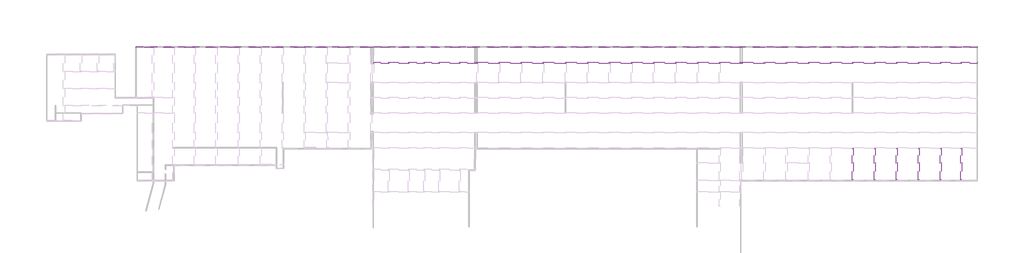
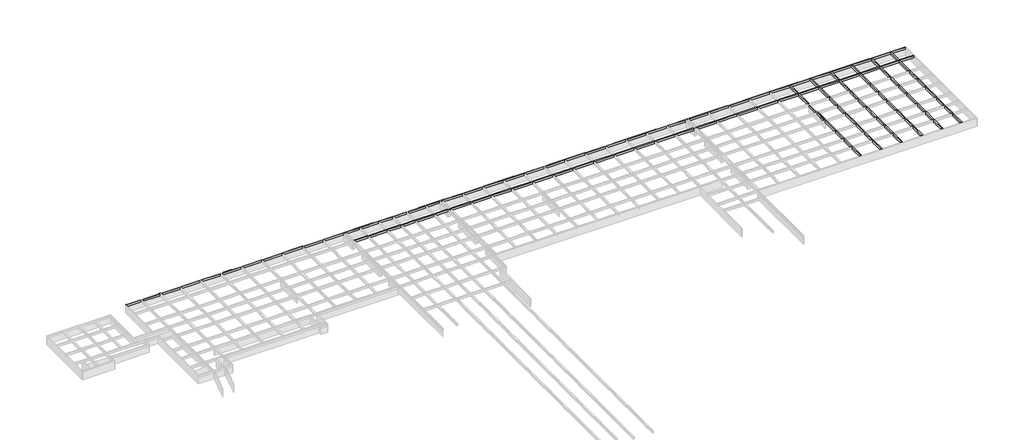
# One storey, part 14 of 14: 8 beams.
"""IFC4 building model written with IfcOpenShell, lengths in millimetres."""

import ifcopenshell
import ifcopenshell.guid

model = None  # the IFC model being written
_history = None  # IfcOwnerHistory: only IFC2X3 demands one
_inside = {}  # id of a spatial element -> (the spatial element, [elements in it])
_under = {}  # id of a project, library or spatial element -> (it, [spatial elements below it])
_declared = {}  # id of a project -> (the project, [libraries it declares])
_typed = {}  # id of a type object -> (the type object, [elements of that type])
_made_of = {}  # id of a material, layer set ... -> (it, [elements and type objects made of it])


def new_model(schema):
    """Start an empty IFC model of exactly this schema.

    Asked for "IFC4X3", IfcOpenShell would pick the latest addendum, in which some entities
    have other attributes; the version numbers below select the first issue.
    IFC2X3 requires an IfcOwnerHistory on every rooted entity: one is made here for all.
    """
    global model, _history
    if schema == "IFC4X3":
        model = ifcopenshell.file(schema_version=(4, 3, 0, 0))
    else:
        model = ifcopenshell.file(schema=schema)
    _inside.clear()
    _under.clear()
    _declared.clear()
    _typed.clear()
    _made_of.clear()
    _history = None
    if model.schema == "IFC2X3":
        org = make("IfcOrganization", Name="unknown")
        user = make(
            "IfcPersonAndOrganization",
            ThePerson=make("IfcPerson", FamilyName="unknown"),
            TheOrganization=org,
        )
        app = make(
            "IfcApplication",
            ApplicationDeveloper=org,
            Version="unknown",
            ApplicationFullName="unknown",
            ApplicationIdentifier="unknown",
        )
        _history = make(
            "IfcOwnerHistory",
            OwningUser=user,
            OwningApplication=app,
            ChangeAction="ADDED",
            CreationDate=0,
        )
    return model


def make(cls, **values):
    """One entity of the class cls with the attributes given. An attribute that is None is left unset."""
    return model.create_entity(
        cls, **{name: value for name, value in values.items() if value is not None}
    )


def rooted(cls, **values):
    """An entity with a GlobalId (a new one), such as an element, a storey or a relation."""
    return make(cls, GlobalId=ifcopenshell.guid.new(), OwnerHistory=_history, **values)


def si_unit(unit_type, name, prefix=None):
    """IfcSIUnit, for example si_unit("LENGTHUNIT", "METRE", prefix="MILLI")."""
    return make("IfcSIUnit", UnitType=unit_type, Prefix=prefix, Name=name)


def assignment(units):
    """IfcUnitAssignment: the units of a project."""
    return None if units is None else make("IfcUnitAssignment", Units=units)


def point(xyz):
    """IfcCartesianPoint."""
    return None if xyz is None else make("IfcCartesianPoint", Coordinates=xyz)


def direction(xyz):
    """IfcDirection."""
    return None if xyz is None else make("IfcDirection", DirectionRatios=xyz)


def frame(location, z_axis=None, x_axis=None):
    """IfcAxis2Placement3D, a coordinate frame: its origin and axes. An axis left out is left unset."""
    return make(
        "IfcAxis2Placement3D",
        Location=point(location),
        Axis=direction(z_axis),
        RefDirection=direction(x_axis),
    )


def origin():
    """The frame at (0, 0, 0) with its axes left unset."""
    return frame((0.0, 0.0, 0.0))


def place(relative_to, where):
    """IfcLocalPlacement: puts the frame where relative to a parent placement (None: the world)."""
    return make(
        "IfcLocalPlacement", PlacementRelTo=relative_to, RelativePlacement=where
    )


def context(
    kind, dimensions, precision=None, world=None, true_north=None, identifier=None
):
    """IfcGeometricRepresentationContext, for example the 3D "Model" context."""
    return make(
        "IfcGeometricRepresentationContext",
        ContextIdentifier=identifier,
        ContextType=kind,
        CoordinateSpaceDimension=dimensions,
        Precision=precision,
        WorldCoordinateSystem=world,
        TrueNorth=true_north,
    )


def project(units=None, contexts=None):
    """IfcProject with its units and contexts."""
    return rooted(
        "IfcProject",
        Name="project",
        RepresentationContexts=contexts,
        UnitsInContext=assignment(units),
    )


def spatial(cls, under=None, at=None, **own):
    """A site, building, storey or space (cls), placed at a placement, below another one or the project."""
    s = rooted(cls, ObjectPlacement=at, **own)
    if under is not None:
        _under.setdefault(under.id(), (under, []))[1].append(s)
    return s


def faces_of(points, faces, orient=None, outer=None):
    """IfcFace entities. A face is a list of loops; a loop is a list of indices into points, from 0.

    orient and outer hold one flag for each loop. By default every Orientation is true, the
    first loop of a face is its IfcFaceOuterBound and the others are IfcFaceBound.
    """
    made = []
    for i, loops in enumerate(faces):
        bounds = []
        for j, loop in enumerate(loops):
            is_outer = j == 0 if outer is None else outer[i][j]
            bounds.append(
                make(
                    "IfcFaceOuterBound" if is_outer else "IfcFaceBound",
                    Bound=make("IfcPolyLoop", Polygon=[points[k] for k in loop]),
                    Orientation=True if orient is None else orient[i][j],
                )
            )
        made.append(make("IfcFace", Bounds=bounds))
    return made


def faceted_brep(points, faces, orient=None, outer=None, voids=None):
    """IfcFacetedBrep: a solid bounded by flat faces; with voids (closed shells), ...WithVoids."""
    shared = [point(p) for p in points]
    hull = make("IfcClosedShell", CfsFaces=faces_of(shared, faces, orient, outer))
    if voids is None:
        return make("IfcFacetedBrep", Outer=hull)
    return make(
        "IfcFacetedBrepWithVoids",
        Outer=hull,
        Voids=[
            make(cls, CfsFaces=faces_of(shared, fs, o, b)) for cls, fs, o, b in voids
        ],
    )


def shape(context_of_items, identifier, shape_type, items):
    """IfcShapeRepresentation: the items that make up one representation, for example the "Body"."""
    return make(
        "IfcShapeRepresentation",
        ContextOfItems=context_of_items,
        RepresentationIdentifier=identifier,
        RepresentationType=shape_type,
        Items=items,
    )


def made_of(thing, what):
    """Note that an element or type object is made of a material, layer set ...; save() writes the relation."""
    if what is not None:
        _made_of.setdefault(what.id(), (what, []))[1].append(thing)
    return thing


def element(
    cls,
    number,
    at=None,
    inside=None,
    cuts=None,
    type_object=None,
    material=None,
    context=None,
    identifier="Body",
    shape_type=None,
    held_by="IfcProductDefinitionShape",
    body=None,
    shapes=None,
    **own,
):
    """One element of the class cls, such as IfcWall. Its Tag is "e" and its number.

    at: its placement. inside: the storey or other place that contains it. cuts: it is an
    opening in that element (IfcRelVoidsElement). A single representation is given by context,
    identifier, shape_type and body (its items); several are given by shapes. held_by: the class
    of the entity that holds the representations. save() writes the other relations.
    """
    e = rooted(cls, Tag="e%d" % number, ObjectPlacement=at, **own)
    if body is not None:
        shapes = [shape(context, identifier, shape_type, body)]
    if shapes is not None:
        e.Representation = make(held_by, Representations=shapes)
    if inside is not None:
        _inside.setdefault(inside.id(), (inside, []))[1].append(e)
    if cuts is not None:
        rooted(
            "IfcRelVoidsElement", RelatingBuildingElement=cuts, RelatedOpeningElement=e
        )
    if type_object is not None:
        _typed.setdefault(type_object.id(), (type_object, []))[1].append(e)
    return made_of(e, material)


def aggregate(whole, parts):
    """IfcRelAggregates: a whole, such as a stair, and the parts it consists of."""
    return rooted("IfcRelAggregates", RelatingObject=whole, RelatedObjects=parts)


def save(model, path):
    """Write the relations noted so far, then the file.

    IfcRelAggregates (storeys below a building ...), IfcRelContainedInSpatialStructure (elements
    in a storey), IfcRelDefinesByType, IfcRelAssociatesMaterial and IfcRelDeclares: one each for
    every whole, place, type object, material and project.
    """
    for whole, parts in _under.values():
        aggregate(whole, parts)
    for where, things in _inside.values():
        rooted(
            "IfcRelContainedInSpatialStructure",
            RelatedElements=things,
            RelatingStructure=where,
        )
    for kind, things in _typed.values():
        rooted("IfcRelDefinesByType", RelatedObjects=things, RelatingType=kind)
    for what, things in _made_of.values():
        rooted("IfcRelAssociatesMaterial", RelatedObjects=things, RelatingMaterial=what)
    for by, libraries in _declared.values():
        rooted("IfcRelDeclares", RelatingContext=by, RelatedDefinitions=libraries)
    model.write(path)


model = new_model("IFC4")

# Units and contexts
model_context = context("Model", 3, world=origin())
ifc_project = project(units=[si_unit("LENGTHUNIT", "METRE", prefix="MILLI")], contexts=[model_context])

# Site, building, storey
site = spatial("IfcSite", under=ifc_project)
building = spatial("IfcBuilding", under=site)
storey = spatial("IfcBuildingStorey", under=building, Name="户型图", Elevation=0.0)

# Beams
placement = place(None, origin())
element("IfcBeam", 1, ObjectType="混凝土 - 矩形梁 : KL_beam", at=placement, inside=storey, context=model_context, shape_type="Brep", body=[
    faceted_brep([(227227.2949044, -122797.8127788, 3300.0), (227227.2949044, -123197.8127788, 3300.0), (227227.2949044, -123197.8127788, 2500.0), (227227.2949044, -122797.8127788, 2500.0), (221727.2949044, -122797.8127788, 3300.0), (221327.2949044, -122797.8127788, 3300.0), (214491.1566028, -122797.8127788, 3300.0), (214091.1566028, -122797.8127788, 3300.0), (206763.3308695, -122797.8127788, 3300.0), (206363.3308695, -122797.8127788, 3300.0), (198949.6658892, -122797.8127788, 3300.0), (198549.6658892, -122797.8127788, 3300.0), (191137.2949044, -122797.8127788, 3300.0), (190737.2949044, -122797.8127788, 3300.0), (183327.7006088, -122797.8127788, 3300.0), (182927.7006088, -122797.8127788, 3300.0), (175558.5232577, -122797.8127788, 3300.0), (175158.5232577, -122797.8127788, 3300.0), (167740.9658811, -122797.8127788, 3300.0), (167340.9658811, -122797.8127788, 3300.0), (159907.8874304, -122797.8127788, 3300.0), (159507.8874304, -122797.8127788, 3300.0), (152140.9658811, -122797.8127788, 3300.0), (151740.9658811, -122797.8127788, 3300.0), (144337.2949044, -122797.8127788, 3300.0), (143937.2949044, -122797.8127788, 3300.0), (143577.2949044, -122797.8127788, 3300.0), (143177.2949044, -122797.8127788, 3300.0), (136347.2949044, -122797.8127788, 3300.0), (135947.2949044, -122797.8127788, 3300.0), (128527.2949044, -122797.8127788, 3300.0), (128127.2949044, -122797.8127788, 3300.0), (120717.7893795, -122797.8127788, 3300.0), (120317.7893795, -122797.8127788, 3300.0), (112927.2949044, -122797.8127788, 3300.0), (112527.2949044, -122797.8127788, 3300.0), (105157.0968236, -122797.8127788, 3300.0), (104757.0968236, -122797.8127788, 3300.0), (97322.1026691, -122797.8127788, 3300.0), (96922.1026691, -122797.8127788, 3300.0), (89602.2949044, -122797.8127788, 3300.0), (89202.2949044, -122797.8127788, 3300.0), (81802.2949044, -122797.8127788, 3300.0), (81402.2949044, -122797.8127788, 3300.0), (73867.4871398, -122797.8127788, 3300.0), (73467.4871398, -122797.8127788, 3300.0), (66130.1134745, -122797.8127788, 3300.0), (65730.1134745, -122797.8127788, 3300.0), (58330.1134745, -122797.8127788, 3300.0), (57930.1134745, -122797.8127788, 3300.0), (50537.2949044, -122797.8127788, 3300.0), (50137.2949044, -122797.8127788, 3300.0), (49716.5330009, -122797.8127788, 3300.0), (49316.5330009, -122797.8127788, 3300.0), (44331.9066405, -122797.8127788, 3300.0), (43931.9066405, -122797.8127788, 3300.0), (37081.5607309, -122797.8127788, 3300.0), (36681.5607309, -122797.8127788, 3300.0), (31751.9066405, -122797.8127788, 3300.0), (31351.9066405, -122797.8127788, 3300.0), (26321.5607309, -122797.8127788, 3300.0), (25921.5607309, -122797.8127788, 3300.0), (19160.0865653, -122797.8127788, 3300.0), (18760.0865653, -122797.8127788, 3300.0), (13677.2949044, -122797.8127788, 3300.0), (13677.2949044, -123197.8127788, 3300.0), (18760.0865653, -123197.8127788, 3300.0), (19160.0865653, -123197.8127788, 3300.0), (25921.5607309, -123197.8127788, 3300.0), (26321.5607309, -123197.8127788, 3300.0), (31351.9066405, -123197.8127788, 3300.0), (31751.9066405, -123197.8127788, 3300.0), (36681.5607309, -123197.8127788, 3300.0), (37081.5607309, -123197.8127788, 3300.0), (43931.9066405, -123197.8127788, 3300.0), (44331.9066405, -123197.8127788, 3300.0), (49316.5330009, -123197.8127788, 3300.0), (49716.5330009, -123197.8127788, 3300.0), (50137.2949044, -123197.8127788, 3300.0), (50537.2949044, -123197.8127788, 3300.0), (57930.1134745, -123197.8127788, 3300.0), (58330.1134745, -123197.8127788, 3300.0), (65730.1134745, -123197.8127788, 3300.0), (66130.1134745, -123197.8127788, 3300.0), (73467.4871398, -123197.8127788, 3300.0), (73867.4871398, -123197.8127788, 3300.0), (81402.2949044, -123197.8127788, 3300.0), (81802.2949044, -123197.8127788, 3300.0), (89202.2949044, -123197.8127788, 3300.0), (89602.2949044, -123197.8127788, 3300.0), (96922.1026691, -123197.8127788, 3300.0), (97322.1026691, -123197.8127788, 3300.0), (104757.0968236, -123197.8127788, 3300.0), (105157.0968236, -123197.8127788, 3300.0), (112527.2949044, -123197.8127788, 3300.0), (112927.2949044, -123197.8127788, 3300.0), (120317.7893795, -123197.8127788, 3300.0), (120717.7893795, -123197.8127788, 3300.0), (128127.2949044, -123197.8127788, 3300.0), (128527.2949044, -123197.8127788, 3300.0), (135947.2949044, -123197.8127788, 3300.0), (136347.2949044, -123197.8127788, 3300.0), (143177.2949044, -123197.8127788, 3300.0), (143577.2949044, -123197.8127788, 3300.0), (143937.2949044, -123197.8127788, 3300.0), (144337.2949044, -123197.8127788, 3300.0), (151740.9658811, -123197.8127788, 3300.0), (152140.9658811, -123197.8127788, 3300.0), (159507.8874304, -123197.8127788, 3300.0), (159907.8874304, -123197.8127788, 3300.0), (167340.9658811, -123197.8127788, 3300.0), (167740.9658811, -123197.8127788, 3300.0), (175158.5232577, -123197.8127788, 3300.0), (175558.5232577, -123197.8127788, 3300.0), (182927.7006088, -123197.8127788, 3300.0), (183327.7006088, -123197.8127788, 3300.0), (190737.2949044, -123197.8127788, 3300.0), (191137.2949044, -123197.8127788, 3300.0), (198549.6658892, -123197.8127788, 3300.0), (198949.6658892, -123197.8127788, 3300.0), (206363.3308695, -123197.8127788, 3300.0), (206763.3308695, -123197.8127788, 3300.0), (214091.1566028, -123197.8127788, 3300.0), (214491.1566028, -123197.8127788, 3300.0), (221327.2949044, -123197.8127788, 3300.0), (221727.2949044, -123197.8127788, 3300.0), (13677.2949044, -123197.8127788, 2500.0), (18760.0865653, -123197.8127788, 2500.0), (19160.0865653, -123197.8127788, 2500.0), (25921.5607309, -123197.8127788, 2500.0), (26321.5607309, -123197.8127788, 2500.0), (31351.9066405, -123197.8127788, 2500.0), (31751.9066405, -123197.8127788, 2500.0), (36681.5607309, -123197.8127788, 2500.0), (37081.5607309, -123197.8127788, 2500.0), (43931.9066405, -123197.8127788, 2500.0), (44331.9066405, -123197.8127788, 2500.0), (49316.5330009, -123197.8127788, 2500.0), (49716.5330009, -123197.8127788, 2500.0), (50137.2949044, -123197.8127788, 2500.0), (50537.2949044, -123197.8127788, 2500.0), (57930.1134745, -123197.8127788, 2500.0), (58330.1134745, -123197.8127788, 2500.0), (65730.1134745, -123197.8127788, 2500.0), (66130.1134745, -123197.8127788, 2500.0), (73467.4871398, -123197.8127788, 2500.0), (73867.4871398, -123197.8127788, 2500.0), (81402.2949044, -123197.8127788, 2500.0), (81802.2949044, -123197.8127788, 2500.0), (89202.2949044, -123197.8127788, 2500.0), (89602.2949044, -123197.8127788, 2500.0), (96922.1026691, -123197.8127788, 2500.0), (97322.1026691, -123197.8127788, 2500.0), (104757.0968236, -123197.8127788, 2500.0), (105157.0968236, -123197.8127788, 2500.0), (112527.2949044, -123197.8127788, 2500.0), (112927.2949044, -123197.8127788, 2500.0), (120317.7893795, -123197.8127788, 2500.0), (120717.7893795, -123197.8127788, 2500.0), (128127.2949044, -123197.8127788, 2500.0), (128527.2949044, -123197.8127788, 2500.0), (135947.2949044, -123197.8127788, 2500.0), (136347.2949044, -123197.8127788, 2500.0), (143177.2949044, -123197.8127788, 2500.0), (143577.2949044, -123197.8127788, 2500.0), (143937.2949044, -123197.8127788, 2500.0), (144337.2949044, -123197.8127788, 2500.0), (151740.9658811, -123197.8127788, 2500.0), (152140.9658811, -123197.8127788, 2500.0), (159507.8874304, -123197.8127788, 2500.0), (159907.8874304, -123197.8127788, 2500.0), (167340.9658811, -123197.8127788, 2500.0), (167740.9658811, -123197.8127788, 2500.0), (175158.5232577, -123197.8127788, 2500.0), (175558.5232577, -123197.8127788, 2500.0), (182927.7006088, -123197.8127788, 2500.0), (183327.7006088, -123197.8127788, 2500.0), (190737.2949044, -123197.8127788, 2500.0), (191137.2949044, -123197.8127788, 2500.0), (198549.6658892, -123197.8127788, 2500.0), (198949.6658892, -123197.8127788, 2500.0), (206363.3308695, -123197.8127788, 2500.0), (206763.3308695, -123197.8127788, 2500.0), (214091.1566028, -123197.8127788, 2500.0), (214491.1566028, -123197.8127788, 2500.0), (221327.2949044, -123197.8127788, 2500.0), (221727.2949044, -123197.8127788, 2500.0), (13677.2949044, -122797.8127788, 2500.0), (18760.0865653, -122797.8127788, 2500.0), (19160.0865653, -122797.8127788, 2500.0), (25921.5607309, -122797.8127788, 2500.0), (26321.5607309, -122797.8127788, 2500.0), (31351.9066405, -122797.8127788, 2500.0), (31751.9066405, -122797.8127788, 2500.0), (36681.5607309, -122797.8127788, 2500.0), (37081.5607309, -122797.8127788, 2500.0), (43931.9066405, -122797.8127788, 2500.0), (44331.9066405, -122797.8127788, 2500.0), (49316.5330009, -122797.8127788, 2500.0), (49716.5330009, -122797.8127788, 2500.0), (50137.2949044, -122797.8127788, 2500.0), (50537.2949044, -122797.8127788, 2500.0), (57930.1134745, -122797.8127788, 2500.0), (58330.1134745, -122797.8127788, 2500.0), (65730.1134745, -122797.8127788, 2500.0), (66130.1134745, -122797.8127788, 2500.0), (73467.4871398, -122797.8127788, 2500.0), (73867.4871398, -122797.8127788, 2500.0), (81402.2949044, -122797.8127788, 2500.0), (81802.2949044, -122797.8127788, 2500.0), (89202.2949044, -122797.8127788, 2500.0), (89602.2949044, -122797.8127788, 2500.0), (96922.1026691, -122797.8127788, 2500.0), (97322.1026691, -122797.8127788, 2500.0), (104757.0968236, -122797.8127788, 2500.0), (105157.0968236, -122797.8127788, 2500.0), (112527.2949044, -122797.8127788, 2500.0), (112927.2949044, -122797.8127788, 2500.0), (120317.7893795, -122797.8127788, 2500.0), (120717.7893795, -122797.8127788, 2500.0), (128127.2949044, -122797.8127788, 2500.0), (128527.2949044, -122797.8127788, 2500.0), (135947.2949044, -122797.8127788, 2500.0), (136347.2949044, -122797.8127788, 2500.0), (143177.2949044, -122797.8127788, 2500.0), (143577.2949044, -122797.8127788, 2500.0), (143937.2949044, -122797.8127788, 2500.0), (144337.2949044, -122797.8127788, 2500.0), (151740.9658811, -122797.8127788, 2500.0), (152140.9658811, -122797.8127788, 2500.0), (159507.8874304, -122797.8127788, 2500.0), (159907.8874304, -122797.8127788, 2500.0), (167340.9658811, -122797.8127788, 2500.0), (167740.9658811, -122797.8127788, 2500.0), (175158.5232577, -122797.8127788, 2500.0), (175558.5232577, -122797.8127788, 2500.0), (182927.7006088, -122797.8127788, 2500.0), (183327.7006088, -122797.8127788, 2500.0), (190737.2949044, -122797.8127788, 2500.0), (191137.2949044, -122797.8127788, 2500.0), (198549.6658892, -122797.8127788, 2500.0), (198949.6658892, -122797.8127788, 2500.0), (206363.3308695, -122797.8127788, 2500.0), (206763.3308695, -122797.8127788, 2500.0), (214091.1566028, -122797.8127788, 2500.0), (214491.1566028, -122797.8127788, 2500.0), (221327.2949044, -122797.8127788, 2500.0), (221727.2949044, -122797.8127788, 2500.0)], [[[0, 1, 2, 3]], [[1, 0, 4, 5, 6, 7, 8, 9, 10, 11, 12, 13, 14, 15, 16, 17, 18, 19, 20, 21, 22, 23, 24, 25, 26, 27, 28, 29, 30, 31, 32, 33, 34, 35, 36, 37, 38, 39, 40, 41, 42, 43, 44, 45, 46, 47, 48, 49, 50, 51, 52, 53, 54, 55, 56, 57, 58, 59, 60, 61, 62, 63, 64, 65, 66, 67, 68, 69, 70, 71, 72, 73, 74, 75, 76, 77, 78, 79, 80, 81, 82, 83, 84, 85, 86, 87, 88, 89, 90, 91, 92, 93, 94, 95, 96, 97, 98, 99, 100, 101, 102, 103, 104, 105, 106, 107, 108, 109, 110, 111, 112, 113, 114, 115, 116, 117, 118, 119, 120, 121, 122, 123, 124, 125]], [[2, 1, 125, 124, 123, 122, 121, 120, 119, 118, 117, 116, 115, 114, 113, 112, 111, 110, 109, 108, 107, 106, 105, 104, 103, 102, 101, 100, 99, 98, 97, 96, 95, 94, 93, 92, 91, 90, 89, 88, 87, 86, 85, 84, 83, 82, 81, 80, 79, 78, 77, 76, 75, 74, 73, 72, 71, 70, 69, 68, 67, 66, 65, 126, 127, 128, 129, 130, 131, 132, 133, 134, 135, 136, 137, 138, 139, 140, 141, 142, 143, 144, 145, 146, 147, 148, 149, 150, 151, 152, 153, 154, 155, 156, 157, 158, 159, 160, 161, 162, 163, 164, 165, 166, 167, 168, 169, 170, 171, 172, 173, 174, 175, 176, 177, 178, 179, 180, 181, 182, 183, 184, 185, 186]], [[3, 2, 186, 185, 184, 183, 182, 181, 180, 179, 178, 177, 176, 175, 174, 173, 172, 171, 170, 169, 168, 167, 166, 165, 164, 163, 162, 161, 160, 159, 158, 157, 156, 155, 154, 153, 152, 151, 150, 149, 148, 147, 146, 145, 144, 143, 142, 141, 140, 139, 138, 137, 136, 135, 134, 133, 132, 131, 130, 129, 128, 127, 126, 187, 188, 189, 190, 191, 192, 193, 194, 195, 196, 197, 198, 199, 200, 201, 202, 203, 204, 205, 206, 207, 208, 209, 210, 211, 212, 213, 214, 215, 216, 217, 218, 219, 220, 221, 222, 223, 224, 225, 226, 227, 228, 229, 230, 231, 232, 233, 234, 235, 236, 237, 238, 239, 240, 241, 242, 243, 244, 245, 246, 247]], [[0, 3, 247, 246, 245, 244, 243, 242, 241, 240, 239, 238, 237, 236, 235, 234, 233, 232, 231, 230, 229, 228, 227, 226, 225, 224, 223, 222, 221, 220, 219, 218, 217, 216, 215, 214, 213, 212, 211, 210, 209, 208, 207, 206, 205, 204, 203, 202, 201, 200, 199, 198, 197, 196, 195, 194, 193, 192, 191, 190, 189, 188, 187, 64, 63, 62, 61, 60, 59, 58, 57, 56, 55, 54, 53, 52, 51, 50, 49, 48, 47, 46, 45, 44, 43, 42, 41, 40, 39, 38, 37, 36, 35, 34, 33, 32, 31, 30, 29, 28, 27, 26, 25, 24, 23, 22, 21, 20, 19, 18, 17, 16, 15, 14, 13, 12, 11, 10, 9, 8, 7, 6, 5, 4]], [[65, 64, 187, 126]]]),
])
element("IfcBeam", 2, ObjectType="混凝土 - 矩形梁 : KL_beam", at=placement, inside=storey, context=model_context, shape_type="Brep", body=[
    faceted_brep([(182927.7006088, -122797.8127788, 3300.0), (183327.7006088, -122797.8127788, 3300.0), (183327.7006088, -117558.950757, 3300.0), (182927.7006088, -117558.950757, 3300.0), (182927.7006088, -122797.8127788, 2500.0), (182927.7006088, -117558.950757, 2500.0), (183327.7006088, -122797.8127788, 2500.0), (183327.7006088, -117558.950757, 2500.0)], [[[0, 1, 2, 3]], [[4, 0, 3, 5]], [[6, 4, 5, 7]], [[1, 6, 7, 2]], [[1, 0, 4, 6]], [[3, 2, 7, 5]]]),
    faceted_brep([(182927.7006088, -123197.8127788, 3300.0), (183327.7006088, -123197.8127788, 3300.0), (183327.7006088, -123197.8127788, 2500.0), (182927.7006088, -123197.8127788, 2500.0), (183327.7006088, -129780.0179086, 3300.0), (182927.7006088, -129780.0179086, 3300.0), (182927.7006088, -129780.0179086, 2500.0), (183327.7006088, -129780.0179086, 2500.0)], [[[0, 1, 2, 3]], [[4, 5, 6, 7]], [[1, 0, 5, 4]], [[0, 3, 6, 5]], [[3, 2, 7, 6]], [[2, 1, 4, 7]]]),
    faceted_brep([(183327.7006088, -130180.0179086, 3300.0), (182927.7006088, -130180.0179086, 3300.0), (182927.7006088, -135180.0179086, 3300.0), (183327.7006088, -135180.0179086, 3300.0), (182927.7006088, -130180.0179086, 2500.0), (182927.7006088, -135180.0179086, 2500.0), (183327.7006088, -130180.0179086, 2500.0), (183327.7006088, -135180.0179086, 2500.0)], [[[0, 1, 2, 3]], [[1, 4, 5, 2]], [[4, 6, 7, 5]], [[6, 0, 3, 7]], [[1, 0, 6, 4]], [[3, 2, 5, 7]]]),
    faceted_brep([(182927.7006088, -135580.0179086, 3300.0), (183327.7006088, -135580.0179086, 3300.0), (183327.7006088, -135580.0179086, 2500.0), (182927.7006088, -135580.0179086, 2500.0), (183327.7006088, -140520.0179086, 3300.0), (182927.7006088, -140520.0179086, 3300.0), (182927.7006088, -140520.0179086, 2500.0), (183327.7006088, -140520.0179086, 2500.0)], [[[0, 1, 2, 3]], [[4, 5, 6, 7]], [[1, 0, 5, 4]], [[0, 3, 6, 5]], [[3, 2, 7, 6]], [[2, 1, 4, 7]]]),
    faceted_brep([(182927.7006088, -140920.0179086, 3300.0), (183327.7006088, -140920.0179086, 3300.0), (183327.7006088, -140920.0179086, 2500.0), (182927.7006088, -140920.0179086, 2500.0), (183327.7006088, -147499.284307, 3300.0), (182927.7006088, -147499.284307, 3300.0), (182927.7006088, -147499.284307, 2500.0), (183327.7006088, -147499.284307, 2500.0)], [[[0, 1, 2, 3]], [[4, 5, 6, 7]], [[1, 0, 5, 4]], [[0, 3, 6, 5]], [[3, 2, 7, 6]], [[2, 1, 4, 7]]]),
    faceted_brep([(182927.7006088, -147899.284307, 3300.0), (183327.7006088, -147899.284307, 3300.0), (183327.7006088, -147899.284307, 2500.0), (182927.7006088, -147899.284307, 2500.0), (183327.7006088, -152899.284307, 3300.0), (182927.7006088, -152899.284307, 3300.0), (182927.7006088, -152899.284307, 2500.0), (183327.7006088, -152899.284307, 2500.0)], [[[0, 1, 2, 3]], [[4, 5, 6, 7]], [[1, 0, 5, 4]], [[0, 3, 6, 5]], [[3, 2, 7, 6]], [[2, 1, 4, 7]]]),
    faceted_brep([(182927.7006088, -153299.284307, 3300.0), (183327.7006088, -153299.284307, 3300.0), (183327.7006088, -153299.284307, 2500.0), (182927.7006088, -153299.284307, 2500.0), (183327.7006088, -164396.0449275, 3300.0), (182927.7006088, -164396.0449275, 3300.0), (182927.7006088, -164396.0449275, 2500.0), (183327.7006088, -164396.0449275, 2500.0), (182927.7006088, -158198.950757, 3300.0), (182927.7006088, -158598.950757, 3300.0), (183327.7006088, -158598.950757, 3300.0), (183327.7006088, -158198.950757, 3300.0), (182927.7006088, -158198.950757, 2500.0), (182927.7006088, -158598.950757, 2500.0), (183327.7006088, -158198.950757, 2500.0), (183327.7006088, -158598.950757, 2500.0)], [[[0, 1, 2, 3]], [[4, 5, 6, 7]], [[1, 0, 8, 9, 5, 4, 10, 11]], [[0, 3, 12, 13, 6, 5, 9, 8]], [[3, 2, 14, 15, 7, 6, 13, 12]], [[2, 1, 11, 10, 4, 7, 15, 14]]]),
])
element("IfcBeam", 3, ObjectType="混凝土 - 矩形梁 : KL_beam", at=placement, inside=storey, context=model_context, shape_type="Brep", body=[
    faceted_brep([(191137.2949044, -153299.284307, 3300.0), (190737.2949044, -153299.284307, 3300.0), (190737.2949044, -158198.950757, 3300.0), (190737.2949044, -158598.950757, 3300.0), (190737.2949044, -164396.0449275, 3300.0), (191137.2949044, -164396.0449275, 3300.0), (191137.2949044, -158598.950757, 3300.0), (191137.2949044, -158198.950757, 3300.0), (191137.2949044, -153299.284307, 2500.0), (191137.2949044, -164396.0449275, 2500.0), (191137.2949044, -158598.950757, 2500.0), (191137.2949044, -158198.950757, 2500.0), (190737.2949044, -153299.284307, 2500.0), (190737.2949044, -164396.0449275, 2500.0), (190737.2949044, -158598.950757, 2500.0), (190737.2949044, -158198.950757, 2500.0)], [[[0, 1, 2, 3, 4, 5, 6, 7]], [[8, 0, 7, 6, 5, 9, 10, 11]], [[12, 8, 11, 10, 9, 13, 14, 15]], [[1, 12, 15, 14, 13, 4, 3, 2]], [[1, 0, 8, 12]], [[5, 4, 13, 9]]]),
    faceted_brep([(190737.2949044, -123197.8127788, 3300.0), (191137.2949044, -123197.8127788, 3300.0), (191137.2949044, -123197.8127788, 2500.0), (190737.2949044, -123197.8127788, 2500.0), (191137.2949044, -129780.0179086, 3300.0), (190737.2949044, -129780.0179086, 3300.0), (190737.2949044, -129780.0179086, 2500.0), (191137.2949044, -129780.0179086, 2500.0)], [[[0, 1, 2, 3]], [[4, 5, 6, 7]], [[1, 0, 5, 4]], [[2, 1, 4, 7]], [[3, 2, 7, 6]], [[0, 3, 6, 5]]]),
    faceted_brep([(191137.2949044, -122797.8127788, 3300.0), (190737.2949044, -122797.8127788, 3300.0), (190737.2949044, -122797.8127788, 2500.0), (191137.2949044, -122797.8127788, 2500.0), (191137.2949044, -117558.950757, 3300.0), (190737.2949044, -117558.950757, 3300.0), (191137.2949044, -117558.950757, 2500.0), (190737.2949044, -117558.950757, 2500.0)], [[[0, 1, 2, 3]], [[1, 0, 4, 5]], [[0, 3, 6, 4]], [[3, 2, 7, 6]], [[2, 1, 5, 7]], [[5, 4, 6, 7]]]),
    faceted_brep([(190737.2949044, -130180.0179086, 3300.0), (191137.2949044, -130180.0179086, 3300.0), (191137.2949044, -130180.0179086, 2500.0), (190737.2949044, -130180.0179086, 2500.0), (191137.2949044, -135180.0179086, 3300.0), (190737.2949044, -135180.0179086, 3300.0), (190737.2949044, -135180.0179086, 2500.0), (191137.2949044, -135180.0179086, 2500.0)], [[[0, 1, 2, 3]], [[4, 5, 6, 7]], [[1, 0, 5, 4]], [[2, 1, 4, 7]], [[3, 2, 7, 6]], [[0, 3, 6, 5]]]),
    faceted_brep([(190737.2949044, -135580.0179086, 3300.0), (191137.2949044, -135580.0179086, 3300.0), (191137.2949044, -135580.0179086, 2500.0), (190737.2949044, -135580.0179086, 2500.0), (191137.2949044, -140520.0179086, 3300.0), (190737.2949044, -140520.0179086, 3300.0), (190737.2949044, -140520.0179086, 2500.0), (191137.2949044, -140520.0179086, 2500.0)], [[[0, 1, 2, 3]], [[4, 5, 6, 7]], [[1, 0, 5, 4]], [[2, 1, 4, 7]], [[3, 2, 7, 6]], [[0, 3, 6, 5]]]),
    faceted_brep([(190737.2949044, -140920.0179086, 3300.0), (191137.2949044, -140920.0179086, 3300.0), (191137.2949044, -140920.0179086, 2500.0), (190737.2949044, -140920.0179086, 2500.0), (191137.2949044, -147499.284307, 3300.0), (190737.2949044, -147499.284307, 3300.0), (190737.2949044, -147499.284307, 2500.0), (191137.2949044, -147499.284307, 2500.0)], [[[0, 1, 2, 3]], [[4, 5, 6, 7]], [[1, 0, 5, 4]], [[2, 1, 4, 7]], [[3, 2, 7, 6]], [[0, 3, 6, 5]]]),
    faceted_brep([(190737.2949044, -147899.284307, 3300.0), (191137.2949044, -147899.284307, 3300.0), (191137.2949044, -147899.284307, 2500.0), (190737.2949044, -147899.284307, 2500.0), (191137.2949044, -152899.284307, 3300.0), (190737.2949044, -152899.284307, 3300.0), (190737.2949044, -152899.284307, 2500.0), (191137.2949044, -152899.284307, 2500.0)], [[[0, 1, 2, 3]], [[4, 5, 6, 7]], [[1, 0, 5, 4]], [[2, 1, 4, 7]], [[3, 2, 7, 6]], [[0, 3, 6, 5]]]),
])
element("IfcBeam", 4, ObjectType="混凝土 - 矩形梁 : KL_beam", at=placement, inside=storey, context=model_context, shape_type="Brep", body=[
    faceted_brep([(198549.6658892, -122797.8127788, 3300.0), (198949.6658892, -122797.8127788, 3300.0), (198949.6658892, -117558.950757, 3300.0), (198549.6658892, -117558.950757, 3300.0), (198549.6658892, -122797.8127788, 2500.0), (198549.6658892, -117558.950757, 2500.0), (198949.6658892, -122797.8127788, 2500.0), (198949.6658892, -117558.950757, 2500.0)], [[[0, 1, 2, 3]], [[4, 0, 3, 5]], [[6, 4, 5, 7]], [[1, 6, 7, 2]], [[1, 0, 4, 6]], [[3, 2, 7, 5]]]),
    faceted_brep([(198549.6658892, -123197.8127788, 3300.0), (198949.6658892, -123197.8127788, 3300.0), (198949.6658892, -123197.8127788, 2500.0), (198549.6658892, -123197.8127788, 2500.0), (198949.6658892, -129780.0179086, 3300.0), (198549.6658892, -129780.0179086, 3300.0), (198549.6658892, -129780.0179086, 2500.0), (198949.6658892, -129780.0179086, 2500.0)], [[[0, 1, 2, 3]], [[4, 5, 6, 7]], [[1, 0, 5, 4]], [[0, 3, 6, 5]], [[3, 2, 7, 6]], [[2, 1, 4, 7]]]),
    faceted_brep([(198949.6658892, -130180.0179086, 3300.0), (198549.6658892, -130180.0179086, 3300.0), (198549.6658892, -135180.0179086, 3300.0), (198949.6658892, -135180.0179086, 3300.0), (198549.6658892, -130180.0179086, 2500.0), (198549.6658892, -135180.0179086, 2500.0), (198949.6658892, -130180.0179086, 2500.0), (198949.6658892, -135180.0179086, 2500.0)], [[[0, 1, 2, 3]], [[1, 4, 5, 2]], [[4, 6, 7, 5]], [[6, 0, 3, 7]], [[1, 0, 6, 4]], [[3, 2, 5, 7]]]),
    faceted_brep([(198549.6658892, -135580.0179086, 3300.0), (198949.6658892, -135580.0179086, 3300.0), (198949.6658892, -135580.0179086, 2500.0), (198549.6658892, -135580.0179086, 2500.0), (198949.6658892, -140520.0179086, 3300.0), (198549.6658892, -140520.0179086, 3300.0), (198549.6658892, -140520.0179086, 2500.0), (198949.6658892, -140520.0179086, 2500.0)], [[[0, 1, 2, 3]], [[4, 5, 6, 7]], [[1, 0, 5, 4]], [[0, 3, 6, 5]], [[3, 2, 7, 6]], [[2, 1, 4, 7]]]),
    faceted_brep([(198549.6658892, -140920.0179086, 3300.0), (198949.6658892, -140920.0179086, 3300.0), (198949.6658892, -140920.0179086, 2500.0), (198549.6658892, -140920.0179086, 2500.0), (198949.6658892, -147499.284307, 3300.0), (198549.6658892, -147499.284307, 3300.0), (198549.6658892, -147499.284307, 2500.0), (198949.6658892, -147499.284307, 2500.0)], [[[0, 1, 2, 3]], [[4, 5, 6, 7]], [[1, 0, 5, 4]], [[0, 3, 6, 5]], [[3, 2, 7, 6]], [[2, 1, 4, 7]]]),
    faceted_brep([(198549.6658892, -147899.284307, 3300.0), (198949.6658892, -147899.284307, 3300.0), (198949.6658892, -147899.284307, 2500.0), (198549.6658892, -147899.284307, 2500.0), (198949.6658892, -152899.284307, 3300.0), (198549.6658892, -152899.284307, 3300.0), (198549.6658892, -152899.284307, 2500.0), (198949.6658892, -152899.284307, 2500.0)], [[[0, 1, 2, 3]], [[4, 5, 6, 7]], [[1, 0, 5, 4]], [[0, 3, 6, 5]], [[3, 2, 7, 6]], [[2, 1, 4, 7]]]),
    faceted_brep([(198549.6658892, -153299.284307, 3300.0), (198949.6658892, -153299.284307, 3300.0), (198949.6658892, -153299.284307, 2500.0), (198549.6658892, -153299.284307, 2500.0), (198949.6658892, -164396.0449275, 3300.0), (198549.6658892, -164396.0449275, 3300.0), (198549.6658892, -164396.0449275, 2500.0), (198949.6658892, -164396.0449275, 2500.0), (198549.6658892, -158198.950757, 3300.0), (198549.6658892, -158598.950757, 3300.0), (198949.6658892, -158598.950757, 3300.0), (198949.6658892, -158198.950757, 3300.0), (198549.6658892, -158198.950757, 2500.0), (198549.6658892, -158598.950757, 2500.0), (198949.6658892, -158198.950757, 2500.0), (198949.6658892, -158598.950757, 2500.0)], [[[0, 1, 2, 3]], [[4, 5, 6, 7]], [[1, 0, 8, 9, 5, 4, 10, 11]], [[0, 3, 12, 13, 6, 5, 9, 8]], [[3, 2, 14, 15, 7, 6, 13, 12]], [[2, 1, 11, 10, 4, 7, 15, 14]]]),
])
element("IfcBeam", 5, ObjectType="混凝土 - 矩形梁 : KL_beam", at=placement, inside=storey, context=model_context, shape_type="Brep", body=[
    faceted_brep([(206763.3308695, -153299.284307, 3300.0), (206363.3308695, -153299.284307, 3300.0), (206363.3308695, -158198.950757, 3300.0), (206363.3308695, -158598.950757, 3300.0), (206363.3308695, -164396.0449275, 3300.0), (206763.3308695, -164396.0449275, 3300.0), (206763.3308695, -158598.950757, 3300.0), (206763.3308695, -158198.950757, 3300.0), (206763.3308695, -153299.284307, 2500.0), (206763.3308695, -164396.0449275, 2500.0), (206763.3308695, -158598.950757, 2500.0), (206763.3308695, -158198.950757, 2500.0), (206363.3308695, -153299.284307, 2500.0), (206363.3308695, -164396.0449275, 2500.0), (206363.3308695, -158598.950757, 2500.0), (206363.3308695, -158198.950757, 2500.0)], [[[0, 1, 2, 3, 4, 5, 6, 7]], [[8, 0, 7, 6, 5, 9, 10, 11]], [[12, 8, 11, 10, 9, 13, 14, 15]], [[1, 12, 15, 14, 13, 4, 3, 2]], [[1, 0, 8, 12]], [[5, 4, 13, 9]]]),
    faceted_brep([(206363.3308695, -123197.8127788, 3300.0), (206763.3308695, -123197.8127788, 3300.0), (206763.3308695, -123197.8127788, 2500.0), (206363.3308695, -123197.8127788, 2500.0), (206763.3308695, -129780.0179086, 3300.0), (206363.3308695, -129780.0179086, 3300.0), (206363.3308695, -129780.0179086, 2500.0), (206763.3308695, -129780.0179086, 2500.0)], [[[0, 1, 2, 3]], [[4, 5, 6, 7]], [[1, 0, 5, 4]], [[2, 1, 4, 7]], [[3, 2, 7, 6]], [[0, 3, 6, 5]]]),
    faceted_brep([(206763.3308695, -122797.8127788, 3300.0), (206363.3308695, -122797.8127788, 3300.0), (206363.3308695, -122797.8127788, 2500.0), (206763.3308695, -122797.8127788, 2500.0), (206763.3308695, -117558.950757, 3300.0), (206363.3308695, -117558.950757, 3300.0), (206763.3308695, -117558.950757, 2500.0), (206363.3308695, -117558.950757, 2500.0)], [[[0, 1, 2, 3]], [[1, 0, 4, 5]], [[0, 3, 6, 4]], [[3, 2, 7, 6]], [[2, 1, 5, 7]], [[5, 4, 6, 7]]]),
    faceted_brep([(206363.3308695, -130180.0179086, 3300.0), (206763.3308695, -130180.0179086, 3300.0), (206763.3308695, -130180.0179086, 2500.0), (206363.3308695, -130180.0179086, 2500.0), (206763.3308695, -135180.0179086, 3300.0), (206363.3308695, -135180.0179086, 3300.0), (206363.3308695, -135180.0179086, 2500.0), (206763.3308695, -135180.0179086, 2500.0)], [[[0, 1, 2, 3]], [[4, 5, 6, 7]], [[1, 0, 5, 4]], [[2, 1, 4, 7]], [[3, 2, 7, 6]], [[0, 3, 6, 5]]]),
    faceted_brep([(206363.3308695, -135580.0179086, 3300.0), (206763.3308695, -135580.0179086, 3300.0), (206763.3308695, -135580.0179086, 2500.0), (206363.3308695, -135580.0179086, 2500.0), (206763.3308695, -140520.0179086, 3300.0), (206363.3308695, -140520.0179086, 3300.0), (206363.3308695, -140520.0179086, 2500.0), (206763.3308695, -140520.0179086, 2500.0)], [[[0, 1, 2, 3]], [[4, 5, 6, 7]], [[1, 0, 5, 4]], [[2, 1, 4, 7]], [[3, 2, 7, 6]], [[0, 3, 6, 5]]]),
    faceted_brep([(206363.3308695, -140920.0179086, 3300.0), (206763.3308695, -140920.0179086, 3300.0), (206763.3308695, -140920.0179086, 2500.0), (206363.3308695, -140920.0179086, 2500.0), (206763.3308695, -147499.284307, 3300.0), (206363.3308695, -147499.284307, 3300.0), (206363.3308695, -147499.284307, 2500.0), (206763.3308695, -147499.284307, 2500.0)], [[[0, 1, 2, 3]], [[4, 5, 6, 7]], [[1, 0, 5, 4]], [[2, 1, 4, 7]], [[3, 2, 7, 6]], [[0, 3, 6, 5]]]),
    faceted_brep([(206363.3308695, -147899.284307, 3300.0), (206763.3308695, -147899.284307, 3300.0), (206763.3308695, -147899.284307, 2500.0), (206363.3308695, -147899.284307, 2500.0), (206763.3308695, -152899.284307, 3300.0), (206363.3308695, -152899.284307, 3300.0), (206363.3308695, -152899.284307, 2500.0), (206763.3308695, -152899.284307, 2500.0)], [[[0, 1, 2, 3]], [[4, 5, 6, 7]], [[1, 0, 5, 4]], [[2, 1, 4, 7]], [[3, 2, 7, 6]], [[0, 3, 6, 5]]]),
])
element("IfcBeam", 6, ObjectType="混凝土 - 矩形梁 : KL_beam", at=placement, inside=storey, context=model_context, shape_type="Brep", body=[
    faceted_brep([(214091.1566028, -122797.8127788, 3300.0), (214491.1566028, -122797.8127788, 3300.0), (214491.1566028, -117558.950757, 3300.0), (214091.1566028, -117558.950757, 3300.0), (214091.1566028, -122797.8127788, 2500.0), (214091.1566028, -117558.950757, 2500.0), (214491.1566028, -122797.8127788, 2500.0), (214491.1566028, -117558.950757, 2500.0)], [[[0, 1, 2, 3]], [[4, 0, 3, 5]], [[6, 4, 5, 7]], [[1, 6, 7, 2]], [[1, 0, 4, 6]], [[3, 2, 7, 5]]]),
    faceted_brep([(214091.1566028, -123197.8127788, 3300.0), (214491.1566028, -123197.8127788, 3300.0), (214491.1566028, -123197.8127788, 2500.0), (214091.1566028, -123197.8127788, 2500.0), (214491.1566028, -129780.0179086, 3300.0), (214091.1566028, -129780.0179086, 3300.0), (214091.1566028, -129780.0179086, 2500.0), (214491.1566028, -129780.0179086, 2500.0)], [[[0, 1, 2, 3]], [[4, 5, 6, 7]], [[1, 0, 5, 4]], [[0, 3, 6, 5]], [[3, 2, 7, 6]], [[2, 1, 4, 7]]]),
    faceted_brep([(214491.1566028, -130180.0179086, 3300.0), (214091.1566028, -130180.0179086, 3300.0), (214091.1566028, -135180.0179086, 3300.0), (214491.1566028, -135180.0179086, 3300.0), (214091.1566028, -130180.0179086, 2500.0), (214091.1566028, -135180.0179086, 2500.0), (214491.1566028, -130180.0179086, 2500.0), (214491.1566028, -135180.0179086, 2500.0)], [[[0, 1, 2, 3]], [[1, 4, 5, 2]], [[4, 6, 7, 5]], [[6, 0, 3, 7]], [[1, 0, 6, 4]], [[3, 2, 5, 7]]]),
    faceted_brep([(214091.1566028, -135580.0179086, 3300.0), (214491.1566028, -135580.0179086, 3300.0), (214491.1566028, -135580.0179086, 2500.0), (214091.1566028, -135580.0179086, 2500.0), (214491.1566028, -140520.0179086, 3300.0), (214091.1566028, -140520.0179086, 3300.0), (214091.1566028, -140520.0179086, 2500.0), (214491.1566028, -140520.0179086, 2500.0)], [[[0, 1, 2, 3]], [[4, 5, 6, 7]], [[1, 0, 5, 4]], [[0, 3, 6, 5]], [[3, 2, 7, 6]], [[2, 1, 4, 7]]]),
    faceted_brep([(214091.1566028, -140920.0179086, 3300.0), (214491.1566028, -140920.0179086, 3300.0), (214491.1566028, -140920.0179086, 2500.0), (214091.1566028, -140920.0179086, 2500.0), (214491.1566028, -147499.284307, 3300.0), (214091.1566028, -147499.284307, 3300.0), (214091.1566028, -147499.284307, 2500.0), (214491.1566028, -147499.284307, 2500.0)], [[[0, 1, 2, 3]], [[4, 5, 6, 7]], [[1, 0, 5, 4]], [[0, 3, 6, 5]], [[3, 2, 7, 6]], [[2, 1, 4, 7]]]),
    faceted_brep([(214091.1566028, -147899.284307, 3300.0), (214491.1566028, -147899.284307, 3300.0), (214491.1566028, -147899.284307, 2500.0), (214091.1566028, -147899.284307, 2500.0), (214491.1566028, -152899.284307, 3300.0), (214091.1566028, -152899.284307, 3300.0), (214091.1566028, -152899.284307, 2500.0), (214491.1566028, -152899.284307, 2500.0)], [[[0, 1, 2, 3]], [[4, 5, 6, 7]], [[1, 0, 5, 4]], [[0, 3, 6, 5]], [[3, 2, 7, 6]], [[2, 1, 4, 7]]]),
    faceted_brep([(214091.1566028, -153299.284307, 3300.0), (214491.1566028, -153299.284307, 3300.0), (214491.1566028, -153299.284307, 2500.0), (214091.1566028, -153299.284307, 2500.0), (214491.1566028, -164396.0449275, 3300.0), (214091.1566028, -164396.0449275, 3300.0), (214091.1566028, -164396.0449275, 2500.0), (214491.1566028, -164396.0449275, 2500.0), (214091.1566028, -158198.950757, 3300.0), (214091.1566028, -158598.950757, 3300.0), (214491.1566028, -158598.950757, 3300.0), (214491.1566028, -158198.950757, 3300.0), (214091.1566028, -158198.950757, 2500.0), (214091.1566028, -158598.950757, 2500.0), (214491.1566028, -158198.950757, 2500.0), (214491.1566028, -158598.950757, 2500.0)], [[[0, 1, 2, 3]], [[4, 5, 6, 7]], [[1, 0, 8, 9, 5, 4, 10, 11]], [[0, 3, 12, 13, 6, 5, 9, 8]], [[3, 2, 14, 15, 7, 6, 13, 12]], [[2, 1, 11, 10, 4, 7, 15, 14]]]),
])
element("IfcBeam", 7, ObjectType="混凝土 - 矩形梁 : KL_beam", at=placement, inside=storey, context=model_context, shape_type="Brep", body=[
    faceted_brep([(221727.2949044, -153299.284307, 3300.0), (221327.2949044, -153299.284307, 3300.0), (221327.2949044, -158198.950757, 3300.0), (221327.2949044, -158598.950757, 3300.0), (221327.2949044, -164396.0449275, 3300.0), (221727.2949044, -164396.0449275, 3300.0), (221727.2949044, -158598.950757, 3300.0), (221727.2949044, -158198.950757, 3300.0), (221727.2949044, -153299.284307, 2500.0), (221727.2949044, -164396.0449275, 2500.0), (221727.2949044, -158598.950757, 2500.0), (221727.2949044, -158198.950757, 2500.0), (221327.2949044, -153299.284307, 2500.0), (221327.2949044, -164396.0449275, 2500.0), (221327.2949044, -158598.950757, 2500.0), (221327.2949044, -158198.950757, 2500.0)], [[[0, 1, 2, 3, 4, 5, 6, 7]], [[8, 0, 7, 6, 5, 9, 10, 11]], [[12, 8, 11, 10, 9, 13, 14, 15]], [[1, 12, 15, 14, 13, 4, 3, 2]], [[1, 0, 8, 12]], [[5, 4, 13, 9]]]),
    faceted_brep([(221327.2949044, -123197.8127788, 3300.0), (221727.2949044, -123197.8127788, 3300.0), (221727.2949044, -123197.8127788, 2500.0), (221327.2949044, -123197.8127788, 2500.0), (221727.2949044, -129780.0179086, 3300.0), (221327.2949044, -129780.0179086, 3300.0), (221327.2949044, -129780.0179086, 2500.0), (221727.2949044, -129780.0179086, 2500.0)], [[[0, 1, 2, 3]], [[4, 5, 6, 7]], [[1, 0, 5, 4]], [[2, 1, 4, 7]], [[3, 2, 7, 6]], [[0, 3, 6, 5]]]),
    faceted_brep([(221727.2949044, -122797.8127788, 3300.0), (221327.2949044, -122797.8127788, 3300.0), (221327.2949044, -122797.8127788, 2500.0), (221727.2949044, -122797.8127788, 2500.0), (221727.2949044, -117558.950757, 3300.0), (221327.2949044, -117558.950757, 3300.0), (221727.2949044, -117558.950757, 2500.0), (221327.2949044, -117558.950757, 2500.0)], [[[0, 1, 2, 3]], [[1, 0, 4, 5]], [[0, 3, 6, 4]], [[3, 2, 7, 6]], [[2, 1, 5, 7]], [[5, 4, 6, 7]]]),
    faceted_brep([(221327.2949044, -130180.0179086, 3300.0), (221727.2949044, -130180.0179086, 3300.0), (221727.2949044, -130180.0179086, 2500.0), (221327.2949044, -130180.0179086, 2500.0), (221727.2949044, -135180.0179086, 3300.0), (221327.2949044, -135180.0179086, 3300.0), (221327.2949044, -135180.0179086, 2500.0), (221727.2949044, -135180.0179086, 2500.0)], [[[0, 1, 2, 3]], [[4, 5, 6, 7]], [[1, 0, 5, 4]], [[2, 1, 4, 7]], [[3, 2, 7, 6]], [[0, 3, 6, 5]]]),
    faceted_brep([(221327.2949044, -135580.0179086, 3300.0), (221727.2949044, -135580.0179086, 3300.0), (221727.2949044, -135580.0179086, 2500.0), (221327.2949044, -135580.0179086, 2500.0), (221727.2949044, -140520.0179086, 3300.0), (221327.2949044, -140520.0179086, 3300.0), (221327.2949044, -140520.0179086, 2500.0), (221727.2949044, -140520.0179086, 2500.0)], [[[0, 1, 2, 3]], [[4, 5, 6, 7]], [[1, 0, 5, 4]], [[2, 1, 4, 7]], [[3, 2, 7, 6]], [[0, 3, 6, 5]]]),
    faceted_brep([(221327.2949044, -140920.0179086, 3300.0), (221727.2949044, -140920.0179086, 3300.0), (221727.2949044, -140920.0179086, 2500.0), (221327.2949044, -140920.0179086, 2500.0), (221727.2949044, -147499.284307, 3300.0), (221327.2949044, -147499.284307, 3300.0), (221327.2949044, -147499.284307, 2500.0), (221727.2949044, -147499.284307, 2500.0)], [[[0, 1, 2, 3]], [[4, 5, 6, 7]], [[1, 0, 5, 4]], [[2, 1, 4, 7]], [[3, 2, 7, 6]], [[0, 3, 6, 5]]]),
    faceted_brep([(221327.2949044, -147899.284307, 3300.0), (221727.2949044, -147899.284307, 3300.0), (221727.2949044, -147899.284307, 2500.0), (221327.2949044, -147899.284307, 2500.0), (221727.2949044, -152899.284307, 3300.0), (221327.2949044, -152899.284307, 3300.0), (221327.2949044, -152899.284307, 2500.0), (221727.2949044, -152899.284307, 2500.0)], [[[0, 1, 2, 3]], [[4, 5, 6, 7]], [[1, 0, 5, 4]], [[2, 1, 4, 7]], [[3, 2, 7, 6]], [[0, 3, 6, 5]]]),
])
element("IfcBeam", 8, ObjectType="混凝土 - 矩形梁 : KL_beam", at=placement, inside=storey, context=model_context, shape_type="Brep", body=[
    faceted_brep([(227227.2949044, -117158.950757, 3300.0), (227227.2949044, -117558.950757, 3300.0), (227227.2949044, -117558.950757, 2500.0), (227227.2949044, -117158.950757, 2500.0), (-70372.7050956, -117158.950757, 3300.0), (-70372.7050956, -117158.950757, 2500.0), (-70372.7050956, -117558.950757, 2500.0), (-70372.7050956, -117558.950757, 3300.0), (-64612.7050956, -117558.950757, 3300.0), (-64212.7050956, -117558.950757, 3300.0), (-57355.3281677, -117558.950757, 3300.0), (-56955.3281677, -117558.950757, 3300.0), (-49869.9201432, -117558.950757, 3300.0), (-49469.9201432, -117558.950757, 3300.0), (-42115.0194088, -117558.950757, 3300.0), (-41715.0194088, -117558.950757, 3300.0), (-34272.7050956, -117558.950757, 3300.0), (-33872.7050956, -117558.950757, 3300.0), (-26492.7050956, -117558.950757, 3300.0), (-26092.7050956, -117558.950757, 3300.0), (-18655.2993912, -117558.950757, 3300.0), (-18255.2993912, -117558.950757, 3300.0), (-10914.1452268, -117558.950757, 3300.0), (-10514.1452268, -117558.950757, 3300.0), (-3091.5778774, -117558.950757, 3300.0), (-2691.5778774, -117558.950757, 3300.0), (4754.7716095, -117558.950757, 3300.0), (5154.7716095, -117558.950757, 3300.0), (12577.2949044, -117558.950757, 3300.0), (12977.2949044, -117558.950757, 3300.0), (13277.2949044, -117558.950757, 3300.0), (13677.2949044, -117558.950757, 3300.0), (18760.0865653, -117558.950757, 3300.0), (19160.0865653, -117558.950757, 3300.0), (25921.5607309, -117558.950757, 3300.0), (26321.5607309, -117558.950757, 3300.0), (31351.9066405, -117558.950757, 3300.0), (31751.9066405, -117558.950757, 3300.0), (36681.5607309, -117558.950757, 3300.0), (37081.5607309, -117558.950757, 3300.0), (43931.9066405, -117558.950757, 3300.0), (44331.9066405, -117558.950757, 3300.0), (49316.5330009, -117558.950757, 3300.0), (49716.5330009, -117558.950757, 3300.0), (50137.2949044, -117558.950757, 3300.0), (50537.2949044, -117558.950757, 3300.0), (57930.1134745, -117558.950757, 3300.0), (58330.1134745, -117558.950757, 3300.0), (65730.1134745, -117558.950757, 3300.0), (66130.1134745, -117558.950757, 3300.0), (73467.4871398, -117558.950757, 3300.0), (73867.4871398, -117558.950757, 3300.0), (81402.2949044, -117558.950757, 3300.0), (81802.2949044, -117558.950757, 3300.0), (89202.2949044, -117558.950757, 3300.0), (89602.2949044, -117558.950757, 3300.0), (96922.1026691, -117558.950757, 3300.0), (97322.1026691, -117558.950757, 3300.0), (104757.0968236, -117558.950757, 3300.0), (105157.0968236, -117558.950757, 3300.0), (112527.2949044, -117558.950757, 3300.0), (112927.2949044, -117558.950757, 3300.0), (120317.7893795, -117558.950757, 3300.0), (120717.7893795, -117558.950757, 3300.0), (128127.2949044, -117558.950757, 3300.0), (128527.2949044, -117558.950757, 3300.0), (135947.2949044, -117558.950757, 3300.0), (136347.2949044, -117558.950757, 3300.0), (143177.2949044, -117558.950757, 3300.0), (143577.2949044, -117558.950757, 3300.0), (143937.2949044, -117558.950757, 3300.0), (144337.2949044, -117558.950757, 3300.0), (151740.9658811, -117558.950757, 3300.0), (152140.9658811, -117558.950757, 3300.0), (159507.8874304, -117558.950757, 3300.0), (159907.8874304, -117558.950757, 3300.0), (167340.9658811, -117558.950757, 3300.0), (167740.9658811, -117558.950757, 3300.0), (175158.5232577, -117558.950757, 3300.0), (175558.5232577, -117558.950757, 3300.0), (182927.7006088, -117558.950757, 3300.0), (183327.7006088, -117558.950757, 3300.0), (190737.2949044, -117558.950757, 3300.0), (191137.2949044, -117558.950757, 3300.0), (198549.6658892, -117558.950757, 3300.0), (198949.6658892, -117558.950757, 3300.0), (206363.3308695, -117558.950757, 3300.0), (206763.3308695, -117558.950757, 3300.0), (214091.1566028, -117558.950757, 3300.0), (214491.1566028, -117558.950757, 3300.0), (221327.2949044, -117558.950757, 3300.0), (221727.2949044, -117558.950757, 3300.0), (-64612.7050956, -117558.950757, 2500.0), (-64212.7050956, -117558.950757, 2500.0), (-57355.3281677, -117558.950757, 2500.0), (-56955.3281677, -117558.950757, 2500.0), (-49869.9201432, -117558.950757, 2500.0), (-49469.9201432, -117558.950757, 2500.0), (-42115.0194088, -117558.950757, 2500.0), (-41715.0194088, -117558.950757, 2500.0), (-34272.7050956, -117558.950757, 2500.0), (-33872.7050956, -117558.950757, 2500.0), (-26492.7050956, -117558.950757, 2500.0), (-26092.7050956, -117558.950757, 2500.0), (-18655.2993912, -117558.950757, 2500.0), (-18255.2993912, -117558.950757, 2500.0), (-10914.1452268, -117558.950757, 2500.0), (-10514.1452268, -117558.950757, 2500.0), (-3091.5778774, -117558.950757, 2500.0), (-2691.5778774, -117558.950757, 2500.0), (4754.7716095, -117558.950757, 2500.0), (5154.7716095, -117558.950757, 2500.0), (12577.2949044, -117558.950757, 2500.0), (12977.2949044, -117558.950757, 2500.0), (13277.2949044, -117558.950757, 2500.0), (13677.2949044, -117558.950757, 2500.0), (18760.0865653, -117558.950757, 2500.0), (19160.0865653, -117558.950757, 2500.0), (25921.5607309, -117558.950757, 2500.0), (26321.5607309, -117558.950757, 2500.0), (31351.9066405, -117558.950757, 2500.0), (31751.9066405, -117558.950757, 2500.0), (36681.5607309, -117558.950757, 2500.0), (37081.5607309, -117558.950757, 2500.0), (43931.9066405, -117558.950757, 2500.0), (44331.9066405, -117558.950757, 2500.0), (49316.5330009, -117558.950757, 2500.0), (49716.5330009, -117558.950757, 2500.0), (50137.2949044, -117558.950757, 2500.0), (50537.2949044, -117558.950757, 2500.0), (57930.1134745, -117558.950757, 2500.0), (58330.1134745, -117558.950757, 2500.0), (65730.1134745, -117558.950757, 2500.0), (66130.1134745, -117558.950757, 2500.0), (73467.4871398, -117558.950757, 2500.0), (73867.4871398, -117558.950757, 2500.0), (81402.2949044, -117558.950757, 2500.0), (81802.2949044, -117558.950757, 2500.0), (89202.2949044, -117558.950757, 2500.0), (89602.2949044, -117558.950757, 2500.0), (96922.1026691, -117558.950757, 2500.0), (97322.1026691, -117558.950757, 2500.0), (104757.0968236, -117558.950757, 2500.0), (105157.0968236, -117558.950757, 2500.0), (112527.2949044, -117558.950757, 2500.0), (112927.2949044, -117558.950757, 2500.0), (120317.7893795, -117558.950757, 2500.0), (120717.7893795, -117558.950757, 2500.0), (128127.2949044, -117558.950757, 2500.0), (128527.2949044, -117558.950757, 2500.0), (135947.2949044, -117558.950757, 2500.0), (136347.2949044, -117558.950757, 2500.0), (143177.2949044, -117558.950757, 2500.0), (143577.2949044, -117558.950757, 2500.0), (143937.2949044, -117558.950757, 2500.0), (144337.2949044, -117558.950757, 2500.0), (151740.9658811, -117558.950757, 2500.0), (152140.9658811, -117558.950757, 2500.0), (159507.8874304, -117558.950757, 2500.0), (159907.8874304, -117558.950757, 2500.0), (167340.9658811, -117558.950757, 2500.0), (167740.9658811, -117558.950757, 2500.0), (175158.5232577, -117558.950757, 2500.0), (175558.5232577, -117558.950757, 2500.0), (182927.7006088, -117558.950757, 2500.0), (183327.7006088, -117558.950757, 2500.0), (190737.2949044, -117558.950757, 2500.0), (191137.2949044, -117558.950757, 2500.0), (198549.6658892, -117558.950757, 2500.0), (198949.6658892, -117558.950757, 2500.0), (206363.3308695, -117558.950757, 2500.0), (206763.3308695, -117558.950757, 2500.0), (214091.1566028, -117558.950757, 2500.0), (214491.1566028, -117558.950757, 2500.0), (221327.2949044, -117558.950757, 2500.0), (221727.2949044, -117558.950757, 2500.0)], [[[0, 1, 2, 3]], [[4, 5, 6, 7]], [[1, 0, 4, 7, 8, 9, 10, 11, 12, 13, 14, 15, 16, 17, 18, 19, 20, 21, 22, 23, 24, 25, 26, 27, 28, 29, 30, 31, 32, 33, 34, 35, 36, 37, 38, 39, 40, 41, 42, 43, 44, 45, 46, 47, 48, 49, 50, 51, 52, 53, 54, 55, 56, 57, 58, 59, 60, 61, 62, 63, 64, 65, 66, 67, 68, 69, 70, 71, 72, 73, 74, 75, 76, 77, 78, 79, 80, 81, 82, 83, 84, 85, 86, 87, 88, 89, 90, 91]], [[2, 1, 91, 90, 89, 88, 87, 86, 85, 84, 83, 82, 81, 80, 79, 78, 77, 76, 75, 74, 73, 72, 71, 70, 69, 68, 67, 66, 65, 64, 63, 62, 61, 60, 59, 58, 57, 56, 55, 54, 53, 52, 51, 50, 49, 48, 47, 46, 45, 44, 43, 42, 41, 40, 39, 38, 37, 36, 35, 34, 33, 32, 31, 30, 29, 28, 27, 26, 25, 24, 23, 22, 21, 20, 19, 18, 17, 16, 15, 14, 13, 12, 11, 10, 9, 8, 7, 6, 92, 93, 94, 95, 96, 97, 98, 99, 100, 101, 102, 103, 104, 105, 106, 107, 108, 109, 110, 111, 112, 113, 114, 115, 116, 117, 118, 119, 120, 121, 122, 123, 124, 125, 126, 127, 128, 129, 130, 131, 132, 133, 134, 135, 136, 137, 138, 139, 140, 141, 142, 143, 144, 145, 146, 147, 148, 149, 150, 151, 152, 153, 154, 155, 156, 157, 158, 159, 160, 161, 162, 163, 164, 165, 166, 167, 168, 169, 170, 171, 172, 173, 174, 175]], [[3, 2, 175, 174, 173, 172, 171, 170, 169, 168, 167, 166, 165, 164, 163, 162, 161, 160, 159, 158, 157, 156, 155, 154, 153, 152, 151, 150, 149, 148, 147, 146, 145, 144, 143, 142, 141, 140, 139, 138, 137, 136, 135, 134, 133, 132, 131, 130, 129, 128, 127, 126, 125, 124, 123, 122, 121, 120, 119, 118, 117, 116, 115, 114, 113, 112, 111, 110, 109, 108, 107, 106, 105, 104, 103, 102, 101, 100, 99, 98, 97, 96, 95, 94, 93, 92, 6, 5]], [[0, 3, 5, 4]]]),
])

save(model, "model.ifc")

# Revit data of these elements
# Type "混凝土 - 矩形梁 : KL_beam"
#   Length [instance default] = 1524 mm
#   b = 400 mm
#   h = 800 mm
#   Structural Material [instance default] = 混凝土 - 现场浇注混凝土
#   Assembly Code = ""
# Elements 1, 2, 3, 4, 5, 6, 7, 8 (IfcBeam, "混凝土 - 矩形梁 : KL_beam")
#   Comments = ""
#   Structural Material = none
#   Phase Created = 新构造
# Materials
#   "混凝土 - 现场浇注混凝土": class "混凝土", colour RGB 192 192 192, transparency 0
